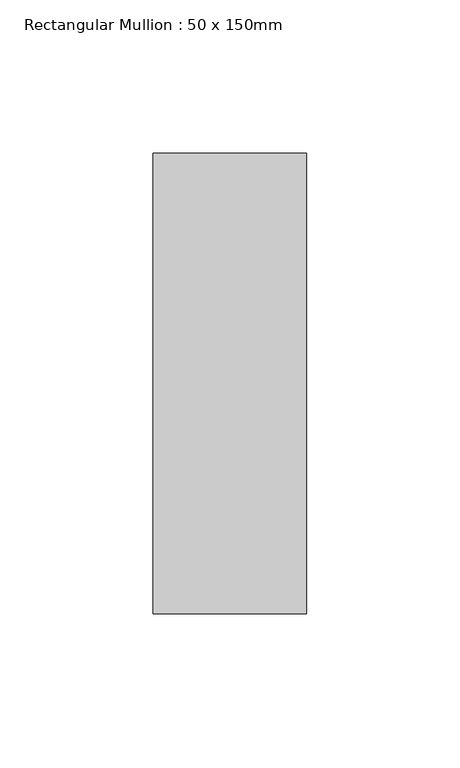
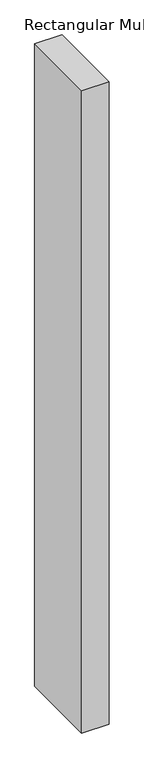
"""IFC4 building model written with IfcOpenShell, lengths in millimetres: member geometry, Rectangular Mullion : 50 x 150mm."""

from ifc_helpers import new_model, si_unit, frame, origin, place, context, project, spatial, polyline, outline, extrude, source, transform, mapped, element, save


def rectangular_mullion_50_x_150mm_8d7ec0e8(model_context):
    return source(origin(), model_context, "Body", "SweptSolid", [
        extrude(outline(polyline([(0.0, 75.0), (0.0, -75.0), (-50.0, -75.0), (-50.0, 75.0), (0.0, 75.0)])), frame((0.0, 0.0, -1250.0000002), z_axis=(0.0, 0.0, 1.0), x_axis=(1.0, 0.0, 0.0)), (0.0, 0.0, 1.0), 1250.0000002),
    ])


if __name__ == "__main__":
    model = new_model("IFC4")
    model_context = context("Model", 3, world=origin())
    ifc_project = project(units=[si_unit("LENGTHUNIT", "METRE", prefix="MILLI")], contexts=[model_context])
    site = spatial("IfcSite", under=ifc_project)
    building = spatial("IfcBuilding", under=site)
    placement = place(None, origin())
    rectangular_mullion_50_x_150mm_shape = rectangular_mullion_50_x_150mm_8d7ec0e8(model_context)
    element("IfcMember", 1, ObjectType="Rectangular Mullion : 50 x 150mm", at=placement, inside=building, context=model_context, shape_type="MappedRepresentation", body=[
        mapped(rectangular_mullion_50_x_150mm_shape, transform((0.0, 0.0, 0.0), x_axis=(1.0, 0.0, 0.0), y_axis=(0.0, 1.0, 0.0), z_axis=(0.0, 0.0, 1.0))),
    ])
    save(model, "model.ifc")

# Revit data of these elements
# Type "Rectangular Mullion : 50 x 150mm"
#   built-in parameter 1007304 = 0.492126 (stored number, unit not read)
#   built-in parameter 1007301 = 0.082021 (stored number, unit not read)
#   built-in parameter 1007300 = 0.082021 (stored number, unit not read)
# Element 1 (IfcMember, "Rectangular Mullion : 50 x 150mm")
#   Materials on its faces: "Aluminium"
# Materials
#   "Aluminium": class "Metal", colour RGB 247 247 247, transparency 0, Description = "Aluminium 6061", Cost = 0
